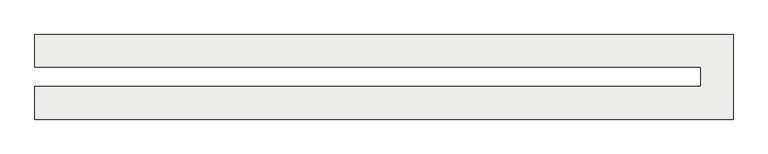
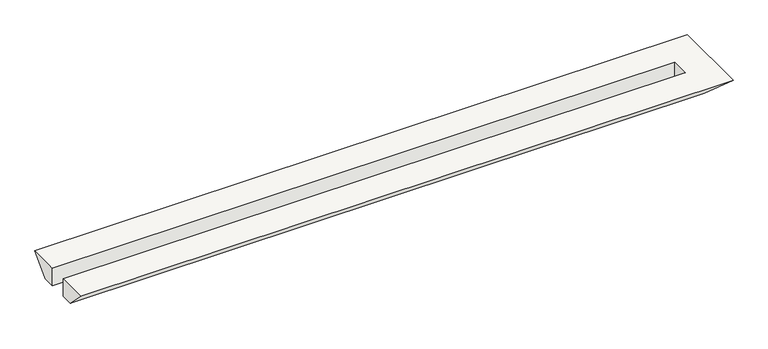
"""IFC4 building model written with IfcOpenShell, lengths in millimetres: slab geometry, Ditch Wall 1 : Ditch Wall 1."""

from ifc_helpers import new_model, si_unit, origin, place, context, project, spatial, faceted_brep, source, transform, mapped, element, save


def slab_cd841ba3(model_context):
    return source(origin(), model_context, "Body", "Brep", [
        faceted_brep([(100.0, 18494.5382614, -200.0), (100.0, 18994.5382614, -200.0), (100.0, 18694.5382614, -500.0), (100.0, 18494.5382614, -500.0), (100.0, 18494.5382614, -300.0), (10325.0, 18494.5382614, -500.0), (10325.0, 18494.5382614, -300.0), (10325.0, 18494.5382614, -200.0), (10325.0, 18194.5382614, -200.0), (100.0, 18194.5382614, -200.0), (100.0, 17694.5382614, -200.0), (10825.0, 17694.5382614, -200.0), (10825.0, 18994.5382614, -200.0), (10525.0, 18694.5382614, -500.0), (10525.0, 17994.5382614, -500.0), (100.0, 17994.5382614, -500.0), (100.0, 18194.5382614, -500.0), (10325.0, 18194.5382614, -500.0), (10325.0, 18194.5382614, -300.0), (100.0, 18194.5382614, -300.0)], [[[0, 1, 2, 3, 4]], [[3, 5, 6, 7, 0, 4]], [[1, 0, 7, 8, 9, 10, 11, 12]], [[2, 1, 12, 13]], [[3, 2, 13, 14, 15, 16, 17, 5]], [[8, 7, 6, 5, 17, 18]], [[13, 12, 11, 14]], [[10, 9, 19, 16, 15]], [[9, 8, 18, 17, 16, 19]], [[15, 14, 11, 10]]]),
    ])


if __name__ == "__main__":
    model = new_model("IFC4")
    model_context = context("Model", 3, world=origin())
    ifc_project = project(units=[si_unit("LENGTHUNIT", "METRE", prefix="MILLI")], contexts=[model_context])
    site = spatial("IfcSite", under=ifc_project)
    building = spatial("IfcBuilding", under=site)
    placement = place(None, origin())
    slab_shape = slab_cd841ba3(model_context)
    element("IfcSlab", 1, ObjectType="Ditch Wall 1 : Ditch Wall 1", at=placement, inside=building, context=model_context, shape_type="MappedRepresentation", body=[
        mapped(slab_shape, transform((0.0, 0.0, 0.0), x_axis=(1.0, 0.0, 0.0), y_axis=(0.0, 1.0, 0.0), z_axis=(0.0, 0.0, 1.0))),
    ])
    save(model, "model.ifc")

# Revit data of these elements
# Element 1 (IfcSlab, "Ditch Wall 1 : Ditch Wall 1")
#   Materials on its faces: "A03AC032-00007_Structural Concrete_Type1_25MPa-30Mpa"
# Materials
#   "A03AC032-00007_Structural Concrete_Type1_25MPa-30Mpa": class "Concrete", colour RGB 176 176 176, transparency 0, Keynote = "09910.A1", Description = "Reinf. Conc.", W00) Work Master Code = "A03AC032-00007", W01) Work Master_Lv1 = "Concrete Work", W02) Work Master_Lv2 = "Substructure Work", W03) Work Master_Spec.1 = "Structural Concrete", W04) Work Master_Spec.2 = "Cement Type-1", W05) Work Master_Spec.3 = "25MPa < F'c (Cylinder Strength) ≤ 30MPa", Cost = 0
